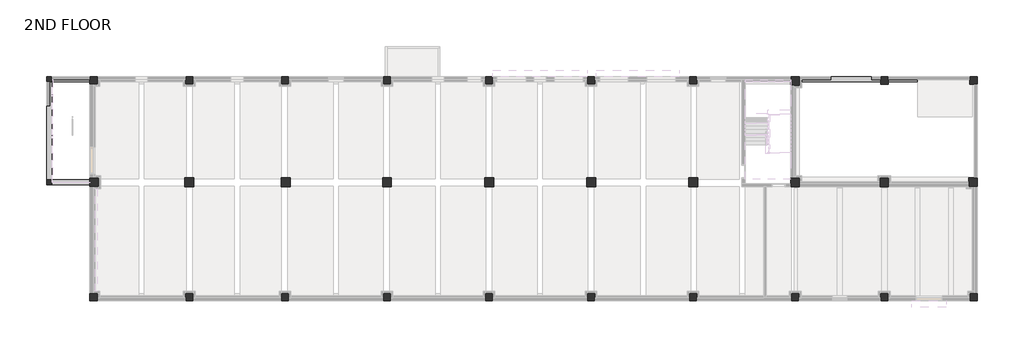
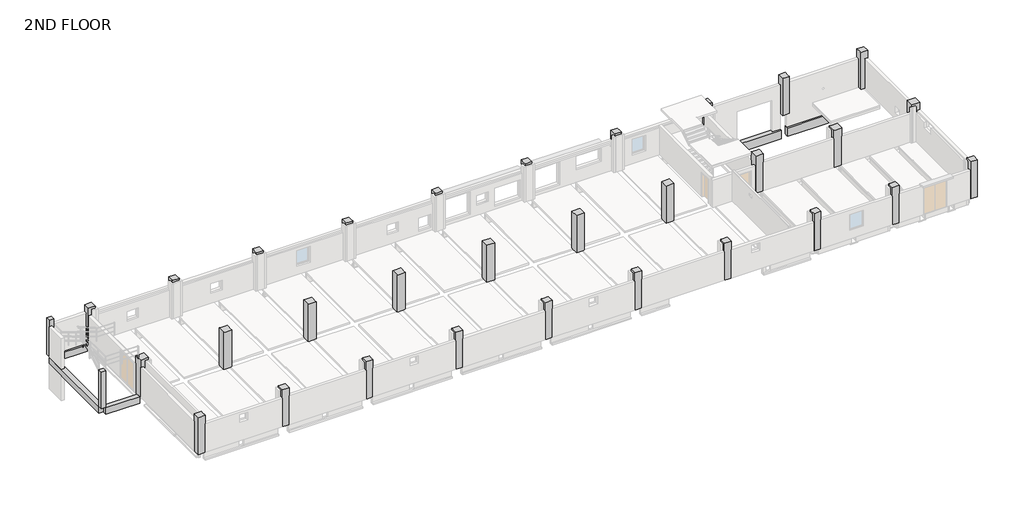
# One storey, part 5 of 7: 32 columns, 8 beams.
"""IFC4 building model written with IfcOpenShell, lengths in millimetres."""

from ifc_helpers import new_model, si_unit, frame, origin, place, context, project, spatial, polyline, outline, extrude, faceted_brep, element, save

model = new_model("IFC4")

# Units and contexts
model_context = context("Model", 3, world=origin())
ifc_project = project(units=[si_unit("LENGTHUNIT", "METRE", prefix="MILLI")], contexts=[model_context])

# Site, building, storey
site = spatial("IfcSite", under=ifc_project)
building = spatial("IfcBuilding", under=site)
storey = spatial("IfcBuildingStorey", under=building, Name="2ND FLOOR", Elevation=10600.0)

# Beams
placement = place(None, origin())
element("IfcBeam", 1, ObjectType="RC Beam_Rectangular : H_SB_AR S16_RC Beam-AG_400x800_2WG1", at=placement, inside=storey, context=model_context, shape_type="Brep", body=[
    faceted_brep([(61700.0, -100.0, 9100.0), (61700.0, 50.0, 9100.0), (61700.0, 300.0, 9100.0), (61000.0, 300.0, 9100.0), (57800.0, 300.0, 9100.0), (55350.0, 300.0, 9100.0), (55350.0, 50.0, 9100.0), (55350.0, -100.0, 9100.0), (61700.0, -100.0, 8300.0), (55350.0, -100.0, 8300.0), (61700.0, 300.0, 8300.0), (61700.0, 50.0, 8300.0), (55350.0, 50.0, 8300.0), (55350.0, 300.0, 8300.0)], [[[0, 1, 2, 3, 4, 5, 6, 7]], [[8, 0, 7, 9]], [[10, 11, 8, 9, 12, 13]], [[2, 10, 13, 5, 4, 3]], [[5, 13, 12, 9, 7, 6]], [[2, 1, 0, 8, 11, 10]]]),
])
element("IfcBeam", 2, ObjectType="RC Beam_Rectangular : H_SB_AR S16_RC Beam-AG_400x800_2WG1", at=placement, inside=storey, context=model_context, shape_type="Brep", body=[
    faceted_brep([(68700.0, -100.0, 9100.0), (68700.0, 50.0, 9100.0), (68700.0, 300.0, 9100.0), (62300.0, 300.0, 9100.0), (62300.0, 50.0, 9100.0), (62300.0, -100.0, 9100.0), (64775.0, -100.0, 9100.0), (64793.0, -100.0, 9100.0), (68700.0, -100.0, 8300.0), (62300.0, -100.0, 8300.0), (64775.0, -100.0, 8300.0), (64793.0, -100.0, 8300.0), (68700.0, 300.0, 8300.0), (68700.0, 50.0, 8300.0), (62300.0, 50.0, 8300.0), (62300.0, 300.0, 8300.0)], [[[0, 1, 2, 3, 4, 5, 6, 7]], [[8, 0, 7, 6, 5, 9, 10, 11]], [[12, 13, 8, 11, 10, 9, 14, 15]], [[2, 12, 15, 3]], [[3, 15, 14, 9, 5, 4]], [[2, 1, 0, 8, 13, 12]]]),
])
element("IfcBeam", 3, ObjectType="RC Beam_Rectangular : H_SB_AR S16_RC Beam-AG_400x600_SWG1", at=placement, inside=storey, context=model_context, shape_type="Brep", body=[
    faceted_brep([(-300.0, -100.0, 10550.0), (-300.0, 50.0, 10550.0), (-300.0, 300.0, 10550.0), (-3300.0, 300.0, 10550.0), (-3300.0, 50.0, 10550.0), (-3300.0, -100.0, 10550.0), (-300.0, -100.0, 9950.0), (-3300.0, -100.0, 9950.0), (-300.0, 300.0, 9950.0), (-300.0, 50.0, 9950.0), (-3300.0, 50.0, 9950.0), (-3300.0, 300.0, 9950.0)], [[[0, 1, 2, 3, 4, 5]], [[6, 0, 5, 7]], [[8, 9, 6, 7, 10, 11]], [[2, 8, 11, 3]], [[2, 1, 0, 6, 9, 8]], [[3, 11, 10, 7, 5, 4]]]),
])
element("IfcBeam", 4, ObjectType="RC Beam_Rectangular : H_SB_AR S16_RC Beam-AG_400x600_SWG2", at=placement, inside=storey, context=model_context, shape_type="Brep", body=[
    faceted_brep([(-3700.0, -7800.0, 10550.0), (-3300.0, -7800.0, 10550.0), (-3300.0, -100.0, 10550.0), (-3450.0, -100.0, 10550.0), (-3700.0, -100.0, 10550.0), (-3700.0, -2000.0, 10550.0), (-3300.0, -7800.0, 9950.0), (-3300.0, -100.0, 9950.0), (-3700.0, -7800.0, 9950.0), (-3700.0, -2000.0, 9950.0), (-3700.0, -100.0, 9950.0), (-3450.0, -100.0, 9950.0)], [[[0, 1, 2, 3, 4, 5]], [[1, 6, 7, 2]], [[6, 8, 9, 10, 11, 7]], [[8, 0, 5, 4, 10, 9]], [[1, 0, 8, 6]], [[4, 3, 2, 7, 11, 10]]]),
])
element("IfcBeam", 5, ObjectType="RC Beam_Rectangular : H_SB_AR S16_RC Beam-AG_400x600_SG1", at=placement, inside=storey, context=model_context, shape_type="SweptSolid", body=[
    extrude(outline(polyline([(-300.0, -7800.0), (-300.0, -8200.0), (-3300.0, -8200.0), (-3300.0, -7800.0), (-300.0, -7800.0)])), frame((0.0, 0.0, 9950.0), z_axis=(0.0, 0.0, 1.0), x_axis=(1.0, 0.0, 0.0)), (0.0, 0.0, 1.0), 600.0),
])
element("IfcBeam", 6, ObjectType="RC Beam_Rectangular : H_SB_AR S16_RC Beam-AG_300x500_2CB1", at=placement, inside=storey, context=model_context, shape_type="Brep", body=[
    faceted_brep([(23150.0, 2350.0, 9300.0), (22850.0, 2350.0, 9300.0), (22850.0, 300.0, 9300.0), (23000.0, 300.0, 9300.0), (23150.0, 300.0, 9300.0), (22850.0, 2350.0, 8800.0), (22850.0, 300.0, 8800.0), (23150.0, 2350.0, 8800.0), (23150.0, 300.0, 8800.0), (23150.0, 2350.0, 9150.0), (23150.0, 300.0, 9150.0)], [[[0, 1, 2, 3, 4]], [[1, 5, 6, 2]], [[5, 7, 8, 6]], [[7, 9, 0, 4, 10, 8]], [[4, 3, 2, 6, 8, 10]], [[0, 9, 7, 5, 1]]]),
])
element("IfcBeam", 7, ObjectType="RC Beam_Rectangular : H_SB_AR S16_RC Beam-AG_300x500_2CB1", at=placement, inside=storey, context=model_context, shape_type="Brep", body=[
    faceted_brep([(27150.0, 2350.0, 9300.0), (26850.0, 2350.0, 9300.0), (26850.0, 300.0, 9300.0), (27000.0, 300.0, 9300.0), (27150.0, 300.0, 9300.0), (26850.0, 2350.0, 9150.0), (26850.0, 2350.0, 8800.0), (26850.0, 300.0, 8800.0), (26850.0, 300.0, 9150.0), (27150.0, 2350.0, 8800.0), (27150.0, 300.0, 8800.0)], [[[0, 1, 2, 3, 4]], [[1, 5, 6, 7, 8, 2]], [[6, 9, 10, 7]], [[9, 0, 4, 10]], [[4, 3, 2, 8, 7, 10]], [[0, 9, 6, 5, 1]]]),
])
element("IfcBeam", 8, ObjectType="RC Beam_Rectangular : H_SB_AR S16_RC Beam-AG_300x500_2CB2", at=placement, inside=storey, context=model_context, shape_type="Brep", body=[
    faceted_brep([(26850.0, 2350.0, 9300.0), (26850.0, 2650.0, 9300.0), (23150.0, 2650.0, 9300.0), (23150.0, 2350.0, 9300.0), (26850.0, 2350.0, 8800.0), (26850.0, 2350.0, 9150.0), (23150.0, 2350.0, 9150.0), (23150.0, 2350.0, 8800.0), (26850.0, 2650.0, 8800.0), (23150.0, 2650.0, 8800.0)], [[[0, 1, 2, 3]], [[4, 5, 0, 3, 6, 7]], [[8, 4, 7, 9]], [[1, 8, 9, 2]], [[2, 9, 7, 6, 3]], [[1, 0, 5, 4, 8]]]),
])

# Columns
element("IfcColumn", 9, ObjectType="RC_Column_Rectangular : H_SC_AR S15_RC Col-AG_700x700_C1", at=placement, inside=storey, context=model_context, shape_type="Brep", body=[
    faceted_brep([(400.0, -7650.0, 10600.0), (400.0, -7700.0, 10600.0), (400.0, -8300.0, 10600.0), (400.0, -8350.0, 10600.0), (399.4974747, -8350.0, 10600.0), (-50.0, -8350.0, 10600.0), (-300.0, -8350.0, 10600.0), (-300.0, -7650.0, 10600.0), (-50.0, -7650.0, 10600.0), (399.4974747, -7650.0, 10600.0), (400.0, -7650.0, 13920.0), (400.0, -7700.0, 13920.0), (400.0, -7700.0, 14100.0), (400.0, -8300.0, 14100.0), (400.0, -8300.0, 13920.0), (400.0, -8350.0, 13920.0), (399.4974747, -8350.0, 13920.0), (399.4974747, -8350.0, 14100.0), (100.0, -8350.0, 14100.0), (-300.0, -8350.0, 14100.0), (-300.0, -8350.0, 13400.0), (-300.0, -7650.0, 14100.0), (-300.0, -7650.0, 13400.0), (100.0, -7650.0, 14100.0), (399.4974747, -7650.0, 14100.0), (399.4974747, -7650.0, 13920.0), (399.4974747, -8300.0, 14100.0), (399.4974747, -7700.0, 14100.0), (399.4974747, -7700.0, 13920.0), (399.4974747, -8300.0, 13920.0)], [[[0, 1, 2, 3, 4, 5, 6, 7, 8, 9]], [[3, 2, 1, 0, 10, 11, 12, 13, 14, 15]], [[6, 5, 4, 3, 15, 16, 17, 18, 19, 20]], [[7, 6, 20, 19, 21, 22]], [[0, 9, 8, 7, 22, 21, 23, 24, 25, 10]], [[21, 19, 18, 17, 26, 13, 12, 27, 24, 23]], [[25, 28, 11, 10]], [[28, 27, 12, 11]], [[28, 25, 24, 27]], [[16, 29, 26, 17]], [[26, 29, 14, 13]], [[29, 16, 15, 14]]]),
])
element("IfcColumn", 10, ObjectType="RC_Column_Rectangular : H_SC_AR S15_RC Col-AG_700x700_C1", at=placement, inside=storey, context=model_context, shape_type="Brep", body=[
    faceted_brep([(7850.0, -7650.0, 10600.0), (7850.0, -8350.0, 10600.0), (7150.0, -8350.0, 10600.0), (7150.0, -7650.0, 10600.0), (7850.0, -7650.0, 13920.0), (7850.0, -7650.0, 14100.0), (7850.0, -7700.0, 14100.0), (7850.0, -8300.0, 14100.0), (7850.0, -8350.0, 14100.0), (7850.0, -8350.0, 13920.0), (7750.0, -8350.0, 14100.0), (7250.0, -8350.0, 14100.0), (7150.0, -8350.0, 14100.0), (7150.0, -8350.0, 13920.0), (7150.0, -8300.0, 14100.0), (7150.0, -7700.0, 14100.0), (7150.0, -7650.0, 14100.0), (7150.0, -7650.0, 13920.0), (7250.0, -7650.0, 14100.0), (7750.0, -7650.0, 14100.0)], [[[0, 1, 2, 3]], [[1, 0, 4, 5, 6, 7, 8, 9]], [[2, 1, 9, 8, 10, 11, 12, 13]], [[3, 2, 13, 12, 14, 15, 16, 17]], [[0, 3, 17, 16, 18, 19, 5, 4]], [[18, 16, 15, 14, 12, 11, 10, 8, 7, 6, 5, 19]]]),
])
element("IfcColumn", 11, ObjectType="RC_Column_Rectangular : H_SC_AR S15_RC Col-AG_700x700_C1", at=placement, inside=storey, context=model_context, shape_type="Brep", body=[
    faceted_brep([(15400.0000001, -7650.0, 10600.0), (15400.0000001, -8350.0, 10600.0), (14700.0000001, -8350.0, 10600.0), (14700.0000001, -7650.0, 10600.0), (15400.0000001, -7650.0, 13920.0), (15400.0000001, -7650.0, 14100.0), (15400.0000001, -7700.0, 14100.0), (15400.0000001, -8300.0, 14100.0), (15400.0000001, -8350.0, 14100.0), (15400.0000001, -8350.0, 13920.0), (15250.0, -8350.0, 14100.0), (14750.0, -8350.0, 14100.0), (14700.0000001, -8350.0, 14100.0), (14700.0000001, -8350.0, 13920.0), (14700.0000001, -8300.0, 14100.0), (14700.0000001, -7700.0, 14100.0), (14700.0000001, -7650.0, 14100.0), (14700.0000001, -7650.0, 13920.0), (14750.0, -7650.0, 14100.0), (15250.0, -7650.0, 14100.0)], [[[0, 1, 2, 3]], [[1, 0, 4, 5, 6, 7, 8, 9]], [[2, 1, 9, 8, 10, 11, 12, 13]], [[3, 2, 13, 12, 14, 15, 16, 17]], [[0, 3, 17, 16, 18, 19, 5, 4]], [[5, 19, 18, 16, 15, 14, 12, 11, 10, 8, 7, 6]]]),
])
element("IfcColumn", 12, ObjectType="RC_Column_Rectangular : H_SC_AR S15_RC Col-AG_700x700_C1", at=placement, inside=storey, context=model_context, shape_type="Brep", body=[
    faceted_brep([(23350.0000003, -7650.0, 10600.0), (23350.0000003, -8350.0, 10600.0), (22650.0000003, -8350.0, 10600.0), (22650.0000003, -7650.0, 10600.0), (23350.0000003, -7650.0, 13920.0), (23350.0000003, -7650.0, 14100.0), (23350.0000003, -7700.0, 14100.0), (23350.0000003, -8300.0, 14100.0), (23350.0000003, -8350.0, 14100.0), (23350.0000003, -8350.0, 13920.0), (23250.0, -8350.0, 14100.0), (22750.0, -8350.0, 14100.0), (22650.0000003, -8350.0, 14100.0), (22650.0000003, -8350.0, 13920.0), (22650.0000003, -8300.0, 14100.0), (22650.0000003, -7700.0, 14100.0), (22650.0000003, -7650.0, 14100.0), (22650.0000003, -7650.0, 13920.0), (22750.0, -7650.0, 14100.0), (23250.0, -7650.0, 14100.0)], [[[0, 1, 2, 3]], [[1, 0, 4, 5, 6, 7, 8, 9]], [[2, 1, 9, 8, 10, 11, 12, 13]], [[3, 2, 13, 12, 14, 15, 16, 17]], [[0, 3, 17, 16, 18, 19, 5, 4]], [[18, 16, 15, 14, 12, 11, 10, 8, 7, 6, 5, 19]]]),
])
element("IfcColumn", 13, ObjectType="RC_Column_Rectangular : H_SC_AR S15_RC Col-AG_700x700_C1", at=placement, inside=storey, context=model_context, shape_type="Brep", body=[
    faceted_brep([(31350.0000002, -7650.0, 10600.0), (31350.0000002, -8350.0, 10600.0), (30650.0000002, -8350.0, 10600.0), (30650.0000002, -7650.0, 10600.0), (31350.0000002, -7650.0, 13920.0), (31350.0000002, -7650.0, 14100.0), (31350.0000002, -7700.0, 14100.0), (31350.0000002, -8300.0, 14100.0), (31350.0000002, -8350.0, 14100.0), (31350.0000002, -8350.0, 13920.0), (31249.9999998, -8350.0, 14100.0), (30750.0000002, -8350.0, 14100.0), (30650.0000002, -8350.0, 14100.0), (30650.0000002, -8350.0, 13920.0), (30650.0000002, -8300.0, 14100.0), (30650.0000002, -7700.0, 14100.0), (30650.0000002, -7650.0, 14100.0), (30650.0000002, -7650.0, 13920.0), (30750.0000002, -7650.0, 14100.0), (31249.9999998, -7650.0, 14100.0)], [[[0, 1, 2, 3]], [[1, 0, 4, 5, 6, 7, 8, 9]], [[2, 1, 9, 8, 10, 11, 12, 13]], [[3, 2, 13, 12, 14, 15, 16, 17]], [[0, 3, 17, 16, 18, 19, 5, 4]], [[18, 16, 15, 14, 12, 11, 10, 8, 7, 6, 5, 19]]]),
])
element("IfcColumn", 14, ObjectType="RC_Column_Rectangular : H_SC_AR S15_RC Col-AG_700x700_C1", at=placement, inside=storey, context=model_context, shape_type="Brep", body=[
    faceted_brep([(39350.0000001, -7650.0, 10600.0), (39350.0000001, -8350.0, 10600.0), (38650.0000001, -8350.0, 10600.0), (38650.0000001, -7650.0, 10600.0), (39350.0000001, -7650.0, 13920.0), (39350.0000001, -7650.0, 14100.0), (39350.0000001, -7700.0, 14100.0), (39350.0000001, -8300.0, 14100.0), (39350.0000001, -8350.0, 14100.0), (39350.0000001, -8350.0, 13920.0), (39249.9999998, -8350.0, 14100.0), (38750.0000002, -8350.0, 14100.0), (38650.0000001, -8350.0, 14100.0), (38650.0000001, -8350.0, 13920.0), (38650.0000001, -8300.0, 14100.0), (38650.0000001, -7700.0, 14100.0), (38650.0000001, -7650.0, 14100.0), (38650.0000001, -7650.0, 13920.0), (38750.0000002, -7650.0, 14100.0), (39249.9999998, -7650.0, 14100.0)], [[[0, 1, 2, 3]], [[1, 0, 4, 5, 6, 7, 8, 9]], [[2, 1, 9, 8, 10, 11, 12, 13]], [[3, 2, 13, 12, 14, 15, 16, 17]], [[0, 3, 17, 16, 18, 19, 5, 4]], [[18, 16, 15, 14, 12, 11, 10, 8, 7, 6, 5, 19]]]),
])
element("IfcColumn", 15, ObjectType="RC_Column_Rectangular : H_SC_AR S15_RC Col-AG_700x700_C1", at=placement, inside=storey, context=model_context, shape_type="Brep", body=[
    faceted_brep([(47349.9999999, -7650.0, 10600.0), (47349.9999999, -8350.0, 10600.0), (46649.9999999, -8350.0, 10600.0), (46649.9999999, -7650.0, 10600.0), (47349.9999999, -7650.0, 13920.0), (47349.9999999, -7650.0, 14100.0), (47349.9999999, -7750.0, 14100.0), (47349.9999999, -8350.0, 14100.0), (47349.9999999, -8350.0, 13920.0), (47250.0, -8350.0, 14100.0), (46750.0, -8350.0, 14100.0), (46649.9999999, -8350.0, 14100.0), (46649.9999999, -8350.0, 13920.0), (46649.9999999, -8300.0, 14100.0), (46649.9999999, -7700.0, 14100.0), (46649.9999999, -7650.0, 14100.0), (46649.9999999, -7650.0, 13920.0), (46750.0, -7650.0, 14100.0), (47250.0, -7650.0, 14100.0)], [[[0, 1, 2, 3]], [[1, 0, 4, 5, 6, 7, 8]], [[2, 1, 8, 7, 9, 10, 11, 12]], [[3, 2, 12, 11, 13, 14, 15, 16]], [[0, 3, 16, 15, 17, 18, 5, 4]], [[17, 15, 14, 13, 11, 10, 9, 7, 6, 5, 18]]]),
])
element("IfcColumn", 16, ObjectType="RC_Column_Rectangular : H_SC_AR S15_RC Col-AG_700x700_C1", at=placement, inside=storey, context=model_context, shape_type="Brep", body=[
    faceted_brep([(55350.0, -7650.0, 10600.0), (55350.0, -8100.0, 10600.0), (55350.0, -8350.0, 10600.0), (54650.0, -8350.0, 10600.0), (54650.0, -8100.0, 10600.0), (54650.0, -7650.0, 10600.0), (54900.0, -7650.0, 10600.0), (55350.0, -7650.0, 13920.0), (55350.0, -7650.0, 14100.0), (55350.0, -7750.0, 14100.0), (55350.0, -8350.0, 14100.0), (55350.0, -8350.0, 13920.0), (55350.0, -8350.0, 13300.0), (55200.0, -8350.0, 14100.0), (54700.0, -8350.0, 14100.0), (54650.0, -8350.0, 14100.0), (54650.0, -8350.0, 13920.0), (54650.0, -8350.0, 13200.0), (54650.0, -7650.0, 14100.0), (54650.0, -7650.0, 13300.0), (55150.0, -7650.0, 14100.0)], [[[0, 1, 2, 3, 4, 5, 6]], [[2, 1, 0, 7, 8, 9, 10, 11, 12]], [[3, 2, 12, 11, 10, 13, 14, 15, 16, 17]], [[5, 4, 3, 17, 16, 15, 18, 19]], [[0, 6, 5, 19, 18, 20, 8, 7]], [[18, 15, 14, 13, 10, 9, 8, 20]]]),
])
element("IfcColumn", 17, ObjectType="RC_Column_Rectangular : H_SC_AR S15_RC Col-AG_700x700_C1", at=placement, inside=storey, context=model_context, shape_type="Brep", body=[
    faceted_brep([(62350.0, -7650.0, 10600.0), (62350.0, -8100.0, 10600.0), (62350.0, -8350.0, 10600.0), (61650.0, -8350.0, 10600.0), (61650.0, -8100.0, 10600.0), (61650.0, -7650.0, 10600.0), (62350.0, -7650.0, 13920.0), (62350.0, -7650.0, 14100.0), (62350.0, -7750.0, 14100.0), (62350.0, -8350.0, 14100.0), (62350.0, -8350.0, 13920.0), (62350.0, -8350.0, 13300.0), (62250.0, -8350.0, 14100.0), (61750.0, -8350.0, 14100.0), (61650.0, -8350.0, 14100.0), (61650.0, -8350.0, 13920.0), (61650.0, -8350.0, 13300.0), (61650.0, -7750.0, 14100.0), (61650.0, -7650.0, 14100.0), (61650.0, -7650.0, 13920.0), (61750.0, -7650.0, 14100.0), (62250.0, -7650.0, 14100.0)], [[[0, 1, 2, 3, 4, 5]], [[2, 1, 0, 6, 7, 8, 9, 10, 11]], [[3, 2, 11, 10, 9, 12, 13, 14, 15, 16]], [[5, 4, 3, 16, 15, 14, 17, 18, 19]], [[0, 5, 19, 18, 20, 21, 7, 6]], [[20, 18, 17, 14, 13, 12, 9, 8, 7, 21]]]),
])
element("IfcColumn", 18, ObjectType="RC_Column_Rectangular : H_SC_AR S15_RC Col-AG_700x700_C1", at=placement, inside=storey, context=model_context, shape_type="Brep", body=[
    faceted_brep([(69300.0, -7650.0, 10600.0), (69300.0, -8350.0, 10600.0), (69050.0, -8350.0, 10600.0), (68600.0, -8350.0, 10600.0), (68600.0, -8100.0, 10600.0), (68600.0, -7650.0, 10600.0), (69050.0, -7650.0, 10600.0), (69300.0, -7650.0, 13400.0), (69300.0, -7650.0, 14100.0), (69300.0, -8350.0, 14100.0), (69300.0, -8350.0, 13400.0), (68900.0, -8350.0, 14100.0), (68600.0, -8350.0, 14100.0), (68600.0, -8350.0, 13920.0), (68600.0, -8350.0, 13300.0), (68600.0, -7750.0, 14100.0), (68600.0, -7650.0, 14100.0), (68600.0, -7650.0, 13920.0), (68900.0, -7650.0, 14100.0)], [[[0, 1, 2, 3, 4, 5, 6]], [[1, 0, 7, 8, 9, 10]], [[3, 2, 1, 10, 9, 11, 12, 13, 14]], [[5, 4, 3, 14, 13, 12, 15, 16, 17]], [[0, 6, 5, 17, 16, 18, 8, 7]], [[9, 8, 18, 16, 15, 12, 11]]]),
])
element("IfcColumn", 19, ObjectType="RC_Column_Rectangular : H_SC_AR S15_RC Col-AG_700x700_C1", at=placement, inside=storey, context=model_context, shape_type="Brep", body=[
    faceted_brep([(55350.0, 300.0, 10600.0), (55350.0, -400.0, 10600.0), (54900.0, -400.0, 10600.0), (54650.0, -400.0, 10600.0), (54650.0, 50.0, 10600.0), (54650.0, 300.0, 10600.0), (55350.0, 300.0, 13300.0), (55350.0, 300.0, 14100.0), (55350.0, -100.0, 14100.0), (55350.0, -400.0, 14100.0), (55350.0, -400.0, 13920.0), (55150.0, -400.0, 14100.0), (54900.0, -400.0, 14100.0), (54650.0, -400.0, 14100.0), (54650.0, -400.0, 13300.0), (54650.0, -387.0, 14100.0), (54650.0, 300.0, 14100.0), (54650.0, 300.0, 13300.0)], [[[0, 1, 2, 3, 4, 5]], [[1, 0, 6, 7, 8, 9, 10]], [[3, 2, 1, 10, 9, 11, 12, 13, 14]], [[5, 4, 3, 14, 13, 15, 16, 17]], [[0, 5, 17, 16, 7, 6]], [[16, 15, 13, 12, 11, 9, 8, 7]]]),
])
element("IfcColumn", 20, ObjectType="RC_Column_Rectangular : H_SC_AR S15_RC Col-AG_600x600_C2", at=placement, inside=storey, context=model_context, shape_type="Brep", body=[
    faceted_brep([(300.0, 300.0, 10600.0), (300.0, 50.0, 10600.0), (300.0, -300.0, 10600.0), (-50.0, -300.0, 10600.0), (-300.0, -300.0, 10600.0), (-300.0, 300.0, 10600.0), (300.0, 300.0, 13300.0), (300.0, 300.0, 14100.0), (300.0, -100.0, 14100.0), (300.0, -300.0, 14100.0), (300.0, -300.0, 13920.0), (100.0, -300.0, 14100.0), (-300.0, -300.0, 14100.0), (-300.0, -300.0, 13400.0), (-300.0, 300.0, 14100.0), (-300.0, 300.0, 14050.0), (-300.0, 300.0, 13450.0)], [[[0, 1, 2, 3, 4, 5]], [[2, 1, 0, 6, 7, 8, 9, 10]], [[4, 3, 2, 10, 9, 11, 12, 13]], [[5, 4, 13, 12, 14, 15, 16]], [[0, 5, 16, 15, 14, 7, 6]], [[14, 12, 11, 9, 8, 7]]]),
])
element("IfcColumn", 21, ObjectType="RC_Column_Rectangular : H_SC_AR S15_RC Col-AG_600x600_C2", at=placement, inside=storey, context=model_context, shape_type="Brep", body=[
    faceted_brep([(7800.0, 300.0, 10600.0), (7800.0, 50.0, 10600.0), (7800.0, -300.0, 10600.0), (7200.0, -300.0, 10600.0), (7200.0, 50.0, 10600.0), (7200.0, 300.0, 10600.0), (7800.0, 300.0, 13300.0), (7800.0, 300.0, 14100.0), (7800.0, -100.0, 14100.0), (7800.0, -300.0, 14100.0), (7800.0, -300.0, 13920.0), (7750.0, -300.0, 14100.0), (7250.0, -300.0, 14100.0), (7200.0, -300.0, 14100.0), (7200.0, -300.0, 13920.0), (7200.0, -100.0, 14100.0), (7200.0, 300.0, 14100.0), (7200.0, 300.0, 13300.0)], [[[0, 1, 2, 3, 4, 5]], [[2, 1, 0, 6, 7, 8, 9, 10]], [[3, 2, 10, 9, 11, 12, 13, 14]], [[5, 4, 3, 14, 13, 15, 16, 17]], [[0, 5, 17, 16, 7, 6]], [[7, 16, 15, 13, 12, 11, 9, 8]]]),
])
element("IfcColumn", 22, ObjectType="RC_Column_Rectangular : H_SC_AR S15_RC Col-AG_600x600_C2", at=placement, inside=storey, context=model_context, shape_type="Brep", body=[
    faceted_brep([(15300.0, 300.0, 10600.0), (15300.0, 50.0, 10600.0), (15300.0, -300.0, 10600.0), (14700.0, -300.0, 10600.0), (14700.0, 50.0, 10600.0), (14700.0, 300.0, 10600.0), (15300.0, 300.0, 13300.0), (15300.0, 300.0, 14100.0), (15300.0, -100.0, 14100.0), (15300.0, -300.0, 14100.0), (15300.0, -300.0, 13920.0), (15250.0, -300.0, 14100.0), (14750.0, -300.0, 14100.0), (14700.0, -300.0, 14100.0), (14700.0, -300.0, 13920.0), (14700.0, -100.0, 14100.0), (14700.0, 300.0, 14100.0), (14700.0, 300.0, 13300.0)], [[[0, 1, 2, 3, 4, 5]], [[2, 1, 0, 6, 7, 8, 9, 10]], [[3, 2, 10, 9, 11, 12, 13, 14]], [[5, 4, 3, 14, 13, 15, 16, 17]], [[0, 5, 17, 16, 7, 6]], [[7, 16, 15, 13, 12, 11, 9, 8]]]),
])
element("IfcColumn", 23, ObjectType="RC_Column_Rectangular : H_SC_AR S15_RC Col-AG_600x600_C2", at=placement, inside=storey, context=model_context, shape_type="Brep", body=[
    faceted_brep([(23300.0, 300.0, 10600.0), (23300.0, 50.0, 10600.0), (23300.0, -300.0, 10600.0), (22700.0, -300.0, 10600.0), (22700.0, 50.0, 10600.0), (22700.0, 300.0, 10600.0), (23300.0, 300.0, 13300.0), (23300.0, 300.0, 14100.0), (23300.0, -100.0, 14100.0), (23300.0, -300.0, 14100.0), (23300.0, -300.0, 13920.0), (23250.0, -300.0, 14100.0), (22750.0, -300.0, 14100.0), (22700.0, -300.0, 14100.0), (22700.0, -300.0, 13920.0), (22700.0, -100.0, 14100.0), (22700.0, 300.0, 14100.0), (22700.0, 300.0, 13300.0)], [[[0, 1, 2, 3, 4, 5]], [[2, 1, 0, 6, 7, 8, 9, 10]], [[3, 2, 10, 9, 11, 12, 13, 14]], [[5, 4, 3, 14, 13, 15, 16, 17]], [[0, 5, 17, 16, 7, 6]], [[7, 16, 15, 13, 12, 11, 9, 8]]]),
])
element("IfcColumn", 24, ObjectType="RC_Column_Rectangular : H_SC_AR S15_RC Col-AG_600x600_C2", at=placement, inside=storey, context=model_context, shape_type="Brep", body=[
    faceted_brep([(31300.0, 300.0, 10600.0), (31300.0, 50.0, 10600.0), (31300.0, -300.0, 10600.0), (30700.0, -300.0, 10600.0), (30700.0, 50.0, 10600.0), (30700.0, 300.0, 10600.0), (31300.0, 300.0, 13300.0), (31300.0, 300.0, 14100.0), (31300.0, -100.0, 14100.0), (31300.0, -300.0, 14100.0), (31300.0, -300.0, 13920.0), (31249.9999998, -300.0, 14100.0), (30750.0000002, -300.0, 14100.0), (30700.0, -300.0, 14100.0), (30700.0, -300.0, 13920.0), (30700.0, -100.0, 14100.0), (30700.0, 300.0, 14100.0), (30700.0, 300.0, 13300.0)], [[[0, 1, 2, 3, 4, 5]], [[2, 1, 0, 6, 7, 8, 9, 10]], [[3, 2, 10, 9, 11, 12, 13, 14]], [[5, 4, 3, 14, 13, 15, 16, 17]], [[0, 5, 17, 16, 7, 6]], [[7, 16, 15, 13, 12, 11, 9, 8]]]),
])
element("IfcColumn", 25, ObjectType="RC_Column_Rectangular : H_SC_AR S15_RC Col-AG_600x600_C2", at=placement, inside=storey, context=model_context, shape_type="Brep", body=[
    faceted_brep([(39300.0, 300.0, 10600.0), (39300.0, 50.0, 10600.0), (39300.0, -300.0, 10600.0), (38700.0, -300.0, 10600.0), (38700.0, 50.0, 10600.0), (38700.0, 300.0, 10600.0), (39300.0, 300.0, 13300.0), (39300.0, 300.0, 14100.0), (39300.0, -100.0, 14100.0), (39300.0, -300.0, 14100.0), (39300.0, -300.0, 13920.0), (39249.9999998, -300.0, 14100.0), (38750.0000002, -300.0, 14100.0), (38700.0, -300.0, 14100.0), (38700.0, -300.0, 13920.0), (38700.0, -100.0, 14100.0), (38700.0, 300.0, 14100.0), (38700.0, 300.0, 13300.0)], [[[0, 1, 2, 3, 4, 5]], [[2, 1, 0, 6, 7, 8, 9, 10]], [[3, 2, 10, 9, 11, 12, 13, 14]], [[5, 4, 3, 14, 13, 15, 16, 17]], [[0, 5, 17, 16, 7, 6]], [[7, 16, 15, 13, 12, 11, 9, 8]]]),
])
element("IfcColumn", 26, ObjectType="RC_Column_Rectangular : H_SC_AR S15_RC Col-AG_600x600_C2", at=placement, inside=storey, context=model_context, shape_type="Brep", body=[
    faceted_brep([(47300.0, 300.0, 10600.0), (47300.0, 50.0, 10600.0), (47300.0, -300.0, 10600.0), (46700.0, -300.0, 10600.0), (46700.0, 50.0, 10600.0), (46700.0, 300.0, 10600.0), (47300.0, 300.0, 13300.0), (47300.0, 300.0, 14100.0), (47300.0, -100.0, 14100.0), (47300.0, -300.0, 14100.0), (47300.0, -300.0, 13920.0), (47250.0, -300.0, 14100.0), (46750.0, -300.0, 14100.0), (46700.0, -300.0, 14100.0), (46700.0, -300.0, 13920.0), (46700.0, -100.0, 14100.0), (46700.0, 300.0, 14100.0), (46700.0, 300.0, 13300.0)], [[[0, 1, 2, 3, 4, 5]], [[2, 1, 0, 6, 7, 8, 9, 10]], [[3, 2, 10, 9, 11, 12, 13, 14]], [[5, 4, 3, 14, 13, 15, 16, 17]], [[0, 5, 17, 16, 7, 6]], [[7, 16, 15, 13, 12, 11, 9, 8]]]),
])
element("IfcColumn", 27, ObjectType="RC_Column_Rectangular : H_SC_AR S15_RC Col-AG_600x600_C2", at=placement, inside=storey, context=model_context, shape_type="Brep", body=[
    faceted_brep([(62300.0, 300.0, 10600.0), (62300.0, -300.0, 10600.0), (61700.0, -300.0, 10600.0), (61700.0, 300.0, 10600.0), (62300.0, 300.0, 13300.0), (62300.0, 300.0, 14100.0), (62300.0, -100.0, 14100.0), (62300.0, -300.0, 14100.0), (62300.0, -300.0, 13920.0), (62250.0, -300.0, 14100.0), (61750.0, -300.0, 14100.0), (61700.0, -300.0, 14100.0), (61700.0, -300.0, 13920.0), (61700.0, -100.0, 14100.0), (61700.0, 300.0, 14100.0), (61700.0, 300.0, 13300.0)], [[[0, 1, 2, 3]], [[1, 0, 4, 5, 6, 7, 8]], [[2, 1, 8, 7, 9, 10, 11, 12]], [[3, 2, 12, 11, 13, 14, 15]], [[0, 3, 15, 14, 5, 4]], [[5, 14, 13, 11, 10, 9, 7, 6]]]),
])
element("IfcColumn", 28, ObjectType="RC_Column_Rectangular : H_SC_AR S15_RC Col-AG_600x600_C2", at=placement, inside=storey, context=model_context, shape_type="Brep", body=[
    faceted_brep([(69300.0, 300.0, 10600.0), (69300.0, -300.0, 10600.0), (69050.0, -300.0, 10600.0), (68700.0, -300.0, 10600.0), (68700.0, 300.0, 10600.0), (69300.0, 300.0, 14100.0), (69300.0, -300.0, 14100.0), (69300.0, -300.0, 13400.0), (68900.0, -300.0, 14100.0), (68700.0, -300.0, 14100.0), (68700.0, -300.0, 13920.0), (68700.0, -100.0, 14100.0), (68700.0, 300.0, 14100.0), (68700.0, 300.0, 13300.0)], [[[0, 1, 2, 3, 4]], [[1, 0, 5, 6, 7]], [[3, 2, 1, 7, 6, 8, 9, 10]], [[4, 3, 10, 9, 11, 12, 13]], [[0, 4, 13, 12, 5]], [[6, 5, 12, 11, 9, 8]]]),
])
element("IfcColumn", 29, ObjectType="RC_Column_Rectangular : H_SC_AR S15_RC Col-AG_600x600_C2", at=placement, inside=storey, context=model_context, shape_type="Brep", body=[
    faceted_brep([(69300.0, -16700.0, 10600.0), (69300.0, -17300.0, 10600.0), (68700.0, -17300.0, 10600.0), (68700.0, -17050.0, 10600.0), (68700.0, -16700.0, 10600.0), (69050.0, -16700.0, 10600.0), (69300.0, -16700.0, 13400.0), (69300.0, -16700.0, 14100.0), (69300.0, -17300.0, 14100.0), (68700.0, -17300.0, 14100.0), (68700.0, -17300.0, 13300.0), (68700.0, -16900.0, 14100.0), (68700.0, -16700.0, 14100.0), (68700.0, -16700.0, 13920.0), (68900.0, -16700.0, 14100.0)], [[[0, 1, 2, 3, 4, 5]], [[1, 0, 6, 7, 8]], [[2, 1, 8, 9, 10]], [[4, 3, 2, 10, 9, 11, 12, 13]], [[0, 5, 4, 13, 12, 14, 7, 6]], [[8, 7, 14, 12, 11, 9]]]),
])
element("IfcColumn", 30, ObjectType="RC_Column_Rectangular : H_SC_AR S15_RC Col-AG_600x600_C2", at=placement, inside=storey, context=model_context, shape_type="Brep", body=[
    faceted_brep([(62300.0, -16700.0, 10600.0), (62300.0, -17050.0, 10600.0), (62300.0, -17300.0, 10600.0), (61700.0, -17300.0, 10600.0), (61700.0, -17050.0, 10600.0), (61700.0, -16700.0, 10600.0), (62300.0, -16700.0, 13920.0), (62300.0, -16700.0, 14100.0), (62300.0, -16900.0, 14100.0), (62300.0, -17300.0, 14100.0), (62300.0, -17300.0, 13300.0), (61700.0, -17300.0, 14100.0), (61700.0, -17300.0, 13300.0), (61700.0, -16900.0, 14100.0), (61700.0, -16700.0, 14100.0), (61700.0, -16700.0, 13920.0), (61750.0, -16700.0, 14100.0), (62250.0, -16700.0, 14100.0)], [[[0, 1, 2, 3, 4, 5]], [[2, 1, 0, 6, 7, 8, 9, 10]], [[3, 2, 10, 9, 11, 12]], [[5, 4, 3, 12, 11, 13, 14, 15]], [[0, 5, 15, 14, 16, 17, 7, 6]], [[11, 9, 8, 7, 17, 16, 14, 13]]]),
])
element("IfcColumn", 31, ObjectType="RC_Column_Rectangular : H_SC_AR S15_RC Col-AG_600x600_C2", at=placement, inside=storey, context=model_context, shape_type="Brep", body=[
    faceted_brep([(55300.0, -16700.0, 10600.0), (55300.0, -17050.0, 10600.0), (55300.0, -17300.0, 10600.0), (54700.0, -17300.0, 10600.0), (54700.0, -17050.0, 10600.0), (54700.0, -16700.0, 10600.0), (55300.0, -16700.0, 13920.0), (55300.0, -16700.0, 14100.0), (55300.0, -16900.0, 14100.0), (55300.0, -17300.0, 14100.0), (55300.0, -17300.0, 13300.0), (54700.0, -17300.0, 14100.0), (54700.0, -17300.0, 13300.0), (54700.0, -16900.0, 14100.0), (54700.0, -16700.0, 14100.0), (54700.0, -16700.0, 13920.0), (55200.0, -16700.0, 14100.0)], [[[0, 1, 2, 3, 4, 5]], [[2, 1, 0, 6, 7, 8, 9, 10]], [[3, 2, 10, 9, 11, 12]], [[5, 4, 3, 12, 11, 13, 14, 15]], [[0, 5, 15, 14, 16, 7, 6]], [[11, 9, 8, 7, 16, 14, 13]]]),
])
element("IfcColumn", 32, ObjectType="RC_Column_Rectangular : H_SC_AR S15_RC Col-AG_600x600_C2", at=placement, inside=storey, context=model_context, shape_type="Brep", body=[
    faceted_brep([(46700.0, -16700.0, 10600.0), (47300.0, -16700.0, 10600.0), (47300.0, -17050.0, 10600.0), (47300.0, -17300.0, 10600.0), (46700.0, -17300.0, 10600.0), (46700.0, -17050.0, 10600.0), (46700.0, -16700.0, 13920.0), (46700.0, -16700.0, 14100.0), (46750.0, -16700.0, 14100.0), (47250.0, -16700.0, 14100.0), (47300.0, -16700.0, 14100.0), (47300.0, -16700.0, 13920.0), (47300.0, -16900.0, 14100.0), (47300.0, -17300.0, 14100.0), (47300.0, -17300.0, 13300.0), (46700.0, -17300.0, 14100.0), (46700.0, -17300.0, 13300.0), (46700.0, -16900.0, 14100.0)], [[[0, 1, 2, 3, 4, 5]], [[1, 0, 6, 7, 8, 9, 10, 11]], [[3, 2, 1, 11, 10, 12, 13, 14]], [[4, 3, 14, 13, 15, 16]], [[0, 5, 4, 16, 15, 17, 7, 6]], [[15, 13, 12, 10, 9, 8, 7, 17]]]),
])
element("IfcColumn", 33, ObjectType="RC_Column_Rectangular : H_SC_AR S15_RC Col-AG_600x600_C2", at=placement, inside=storey, context=model_context, shape_type="Brep", body=[
    faceted_brep([(38700.0, -16700.0, 10600.0), (39300.0, -16700.0, 10600.0), (39300.0, -17050.0, 10600.0), (39300.0, -17300.0, 10600.0), (38700.0, -17300.0, 10600.0), (38700.0, -17050.0, 10600.0), (38700.0, -16700.0, 13920.0), (38700.0, -16700.0, 14100.0), (38750.0000002, -16700.0, 14100.0), (39249.9999998, -16700.0, 14100.0), (39300.0, -16700.0, 14100.0), (39300.0, -16700.0, 13920.0), (39300.0, -16900.0, 14100.0), (39300.0, -17300.0, 14100.0), (39300.0, -17300.0, 13300.0), (38700.0, -17300.0, 14100.0), (38700.0, -17300.0, 13300.0), (38700.0, -16900.0, 14100.0)], [[[0, 1, 2, 3, 4, 5]], [[1, 0, 6, 7, 8, 9, 10, 11]], [[3, 2, 1, 11, 10, 12, 13, 14]], [[4, 3, 14, 13, 15, 16]], [[0, 5, 4, 16, 15, 17, 7, 6]], [[15, 13, 12, 10, 9, 8, 7, 17]]]),
])
element("IfcColumn", 34, ObjectType="RC_Column_Rectangular : H_SC_AR S15_RC Col-AG_600x600_C2", at=placement, inside=storey, context=model_context, shape_type="Brep", body=[
    faceted_brep([(30700.0, -16700.0, 10600.0), (31300.0, -16700.0, 10600.0), (31300.0, -17050.0, 10600.0), (31300.0, -17300.0, 10600.0), (30700.0, -17300.0, 10600.0), (30700.0, -17050.0, 10600.0), (30700.0, -16700.0, 13920.0), (30700.0, -16700.0, 14100.0), (30750.0000002, -16700.0, 14100.0), (31249.9999998, -16700.0, 14100.0), (31300.0, -16700.0, 14100.0), (31300.0, -16700.0, 13920.0), (31300.0, -16900.0, 14100.0), (31300.0, -17300.0, 14100.0), (31300.0, -17300.0, 13300.0), (30700.0, -17300.0, 14100.0), (30700.0, -17300.0, 13300.0), (30700.0, -16900.0, 14100.0)], [[[0, 1, 2, 3, 4, 5]], [[1, 0, 6, 7, 8, 9, 10, 11]], [[3, 2, 1, 11, 10, 12, 13, 14]], [[4, 3, 14, 13, 15, 16]], [[0, 5, 4, 16, 15, 17, 7, 6]], [[15, 13, 12, 10, 9, 8, 7, 17]]]),
])
element("IfcColumn", 35, ObjectType="RC_Column_Rectangular : H_SC_AR S15_RC Col-AG_600x600_C2", at=placement, inside=storey, context=model_context, shape_type="Brep", body=[
    faceted_brep([(22700.0, -16700.0, 10600.0), (23300.0, -16700.0, 10600.0), (23300.0, -17050.0, 10600.0), (23300.0, -17300.0, 10600.0), (22700.0, -17300.0, 10600.0), (22700.0, -17050.0, 10600.0), (22700.0, -16700.0, 13920.0), (22700.0, -16700.0, 14100.0), (22750.0, -16700.0, 14100.0), (23250.0, -16700.0, 14100.0), (23300.0, -16700.0, 14100.0), (23300.0, -16700.0, 13920.0), (23300.0, -16900.0, 14100.0), (23300.0, -17300.0, 14100.0), (23300.0, -17300.0, 13300.0), (22700.0, -17300.0, 14100.0), (22700.0, -17300.0, 13300.0), (22700.0, -16900.0, 14100.0)], [[[0, 1, 2, 3, 4, 5]], [[1, 0, 6, 7, 8, 9, 10, 11]], [[3, 2, 1, 11, 10, 12, 13, 14]], [[4, 3, 14, 13, 15, 16]], [[0, 5, 4, 16, 15, 17, 7, 6]], [[15, 13, 12, 10, 9, 8, 7, 17]]]),
])
element("IfcColumn", 36, ObjectType="RC_Column_Rectangular : H_SC_AR S15_RC Col-AG_600x600_C2", at=placement, inside=storey, context=model_context, shape_type="Brep", body=[
    faceted_brep([(14700.0, -16700.0, 10600.0), (15300.0, -16700.0, 10600.0), (15300.0, -17050.0, 10600.0), (15300.0, -17300.0, 10600.0), (14700.0, -17300.0, 10600.0), (14700.0, -17050.0, 10600.0), (14700.0, -16700.0, 13920.0), (14700.0, -16700.0, 14100.0), (14750.0, -16700.0, 14100.0), (15250.0, -16700.0, 14100.0), (15300.0, -16700.0, 14100.0), (15300.0, -16700.0, 13920.0), (15300.0, -16900.0, 14100.0), (15300.0, -17300.0, 14100.0), (15300.0, -17300.0, 13300.0), (14700.0, -17300.0, 14100.0), (14700.0, -17300.0, 13300.0), (14700.0, -16900.0, 14100.0)], [[[0, 1, 2, 3, 4, 5]], [[1, 0, 6, 7, 8, 9, 10, 11]], [[3, 2, 1, 11, 10, 12, 13, 14]], [[4, 3, 14, 13, 15, 16]], [[0, 5, 4, 16, 15, 17, 7, 6]], [[15, 13, 12, 10, 9, 8, 7, 17]]]),
])
element("IfcColumn", 37, ObjectType="RC_Column_Rectangular : H_SC_AR S15_RC Col-AG_600x600_C2", at=placement, inside=storey, context=model_context, shape_type="Brep", body=[
    faceted_brep([(7200.0, -16700.0, 10600.0), (7800.0, -16700.0, 10600.0), (7800.0, -17050.0, 10600.0), (7800.0, -17300.0, 10600.0), (7200.0, -17300.0, 10600.0), (7200.0, -17050.0, 10600.0), (7200.0, -16700.0, 13920.0), (7200.0, -16700.0, 14100.0), (7250.0, -16700.0, 14100.0), (7750.0, -16700.0, 14100.0), (7800.0, -16700.0, 14100.0), (7800.0, -16700.0, 13920.0), (7800.0, -16900.0, 14100.0), (7800.0, -17300.0, 14100.0), (7800.0, -17300.0, 13300.0), (7200.0, -17300.0, 14100.0), (7200.0, -17300.0, 13300.0), (7200.0, -16900.0, 14100.0)], [[[0, 1, 2, 3, 4, 5]], [[1, 0, 6, 7, 8, 9, 10, 11]], [[3, 2, 1, 11, 10, 12, 13, 14]], [[4, 3, 14, 13, 15, 16]], [[0, 5, 4, 16, 15, 17, 7, 6]], [[15, 13, 12, 10, 9, 8, 7, 17]]]),
])
element("IfcColumn", 38, ObjectType="RC_Column_Rectangular : H_SC_AR S15_RC Col-AG_600x600_C2", at=placement, inside=storey, context=model_context, shape_type="Brep", body=[
    faceted_brep([(-300.0, -16700.0, 10600.0), (-50.0, -16700.0, 10600.0), (300.0, -16700.0, 10600.0), (300.0, -17050.0, 10600.0), (300.0, -17300.0, 10600.0), (-300.0, -17300.0, 10600.0), (-300.0, -16700.0, 13400.0), (-300.0, -16700.0, 14100.0), (100.0, -16700.0, 14100.0), (300.0, -16700.0, 14100.0), (300.0, -16700.0, 13920.0), (300.0, -16900.0, 14100.0), (300.0, -17300.0, 14100.0), (300.0, -17300.0, 13300.0), (-300.0, -17300.0, 14100.0)], [[[0, 1, 2, 3, 4, 5]], [[2, 1, 0, 6, 7, 8, 9, 10]], [[4, 3, 2, 10, 9, 11, 12, 13]], [[5, 4, 13, 12, 14]], [[0, 5, 14, 7, 6]], [[14, 12, 11, 9, 8, 7]]]),
])
element("IfcColumn", 39, ObjectType="RC_Column_Rectangular : H_SC_AR S15_RC Col-AG_400x400_C3", at=placement, inside=storey, context=model_context, shape_type="Brep", body=[
    faceted_brep([(-3300.0, -7800.0, 10600.0), (-3300.0, -8200.0, 10600.0), (-3700.0, -8200.0, 10600.0), (-3700.0, -7800.0, 10600.0), (-3300.0, -7800.0, 14050.0), (-3300.0, -8200.0, 14050.0), (-3300.0, -7800.0, 13450.0), (-3700.0, -8200.0, 14050.0), (-3700.0, -7800.0, 14050.0), (-3700.0, -7800.0, 13450.0)], [[[0, 1, 2, 3]], [[4, 5, 1, 0, 6]], [[5, 7, 2, 1]], [[7, 8, 9, 3, 2]], [[8, 4, 6, 0, 3, 9]], [[4, 8, 7, 5]]]),
])
element("IfcColumn", 40, ObjectType="RC_Column_Rectangular : H_SC_AR S15_RC Col-AG_400x400_C3", at=placement, inside=storey, context=model_context, shape_type="Brep", body=[
    faceted_brep([(-3300.0, 300.0, 10600.0), (-3300.0, -100.0, 10600.0), (-3700.0, -100.0, 10600.0), (-3700.0, 300.0, 10600.0), (-3300.0, 300.0, 14050.0), (-3300.0, -100.0, 14050.0), (-3300.0, -100.0, 13450.0), (-3300.0, 300.0, 13450.0), (-3700.0, -100.0, 14050.0), (-3700.0, -100.0, 13450.0), (-3700.0, 300.0, 14050.0)], [[[0, 1, 2, 3]], [[4, 5, 6, 1, 0, 7]], [[5, 8, 9, 2, 1, 6]], [[8, 10, 3, 2, 9]], [[10, 4, 7, 0, 3]], [[4, 10, 8, 5]]]),
])

save(model, "model.ifc")

# Revit data of these elements
# Type "RC Beam_Rectangular : H_SB_AR S16_RC Beam-AG_400x800_2WG1"
#   Type Comments = "CV-AG"
#   중앙부 하부근 = ""
#   중앙부 상부근 = ""
#   중앙부 보조근 = ""
#   중앙부 늑근 = ""
#   외단부 하부근 = ""
#   외단부 상부근 = ""
#   외단부 보조근 = ""
#   외단부 늑근 = ""
#   부호 = "TG3"
#   내단부 하부근 = ""
#   내단부 상부근 = ""
#   내단부 보조근 = ""
#   내단부 늑근 = ""
#   ALL 하부근 = "3-D20"
#   ALL 상부근 = "3-D20"
#   ALL 보조근 = ""
#   ALL 늑근 = "2-D10 @120"
#   H_Rebar Ratio = 0.14
#   Width = 400 mm
#   Height = 800 mm
#   Length [instance default] = 1524 mm
#   b = 400 mm
#   h = 800 mm
#   hec_material3 [instance default] = none
#   hec_material2 [instance default] = none
#   hec_material1 [instance default] = none
#   Structural Material [instance default] = none
#   Assembly Code = ""
# Type "RC Beam_Rectangular : H_SB_AR S16_RC Beam-AG_400x600_SWG1"
#   Type Comments = "CV-AG"
#   중앙부 하부근 = ""
#   중앙부 상부근 = ""
#   중앙부 보조근 = ""
#   중앙부 늑근 = ""
#   외단부 하부근 = ""
#   외단부 상부근 = ""
#   외단부 보조근 = ""
#   외단부 늑근 = ""
#   부호 = "TG3"
#   내단부 하부근 = ""
#   내단부 상부근 = ""
#   내단부 보조근 = ""
#   내단부 늑근 = ""
#   ALL 하부근 = "3-D20"
#   ALL 상부근 = "3-D20"
#   ALL 보조근 = ""
#   ALL 늑근 = "2-D10 @120"
#   H_Rebar Ratio = 0.14
#   Width = 400 mm
#   Height = 600 mm
#   Length [instance default] = 1524 mm
#   b = 400 mm
#   h = 600 mm
#   hec_material3 [instance default] = none
#   hec_material2 [instance default] = none
#   hec_material1 [instance default] = none
#   Structural Material [instance default] = none
#   Assembly Code = ""
# Type "RC Beam_Rectangular : H_SB_AR S16_RC Beam-AG_400x600_SWG2"
#   Type Comments = "CV-AG"
#   중앙부 하부근 = ""
#   중앙부 상부근 = ""
#   중앙부 보조근 = ""
#   중앙부 늑근 = ""
#   외단부 하부근 = ""
#   외단부 상부근 = ""
#   외단부 보조근 = ""
#   외단부 늑근 = ""
#   부호 = "TG3"
#   내단부 하부근 = ""
#   내단부 상부근 = ""
#   내단부 보조근 = ""
#   내단부 늑근 = ""
#   ALL 하부근 = "3-D20"
#   ALL 상부근 = "3-D20"
#   ALL 보조근 = ""
#   ALL 늑근 = "2-D10 @120"
#   H_Rebar Ratio = 0.14
#   Width = 400 mm
#   Height = 600 mm
#   Length [instance default] = 1524 mm
#   b = 400 mm
#   h = 600 mm
#   hec_material3 [instance default] = none
#   hec_material2 [instance default] = none
#   hec_material1 [instance default] = none
#   Structural Material [instance default] = none
#   Assembly Code = ""
# Type "RC Beam_Rectangular : H_SB_AR S16_RC Beam-AG_400x600_SG1"
#   Type Comments = "CV-AG"
#   중앙부 하부근 = ""
#   중앙부 상부근 = ""
#   중앙부 보조근 = ""
#   중앙부 늑근 = ""
#   외단부 하부근 = ""
#   외단부 상부근 = ""
#   외단부 보조근 = ""
#   외단부 늑근 = ""
#   부호 = "TG3"
#   내단부 하부근 = ""
#   내단부 상부근 = ""
#   내단부 보조근 = ""
#   내단부 늑근 = ""
#   ALL 하부근 = "3-D20"
#   ALL 상부근 = "3-D20"
#   ALL 보조근 = ""
#   ALL 늑근 = "2-D10 @120"
#   H_Rebar Ratio = 0.14
#   Width = 400 mm
#   Height = 600 mm
#   Length [instance default] = 1524 mm
#   b = 400 mm
#   h = 600 mm
#   hec_material3 [instance default] = none
#   hec_material2 [instance default] = none
#   hec_material1 [instance default] = none
#   Structural Material [instance default] = none
#   Assembly Code = ""
# Type "RC Beam_Rectangular : H_SB_AR S16_RC Beam-AG_300x500_2CB1"
#   Type Comments = "CV-AG"
#   중앙부 하부근 = ""
#   중앙부 상부근 = ""
#   중앙부 보조근 = ""
#   중앙부 늑근 = ""
#   외단부 하부근 = ""
#   외단부 상부근 = ""
#   외단부 보조근 = ""
#   외단부 늑근 = ""
#   부호 = "TG3"
#   내단부 하부근 = ""
#   내단부 상부근 = ""
#   내단부 보조근 = ""
#   내단부 늑근 = ""
#   ALL 하부근 = "3-D20"
#   ALL 상부근 = "3-D20"
#   ALL 보조근 = ""
#   ALL 늑근 = "2-D10 @120"
#   H_Rebar Ratio = 0.14
#   Width = 300 mm
#   Height = 500 mm
#   Length [instance default] = 1524 mm
#   b = 300 mm
#   h = 500 mm
#   hec_material3 [instance default] = none
#   hec_material2 [instance default] = none
#   hec_material1 [instance default] = none
#   Structural Material [instance default] = none
#   Assembly Code = ""
# Type "RC Beam_Rectangular : H_SB_AR S16_RC Beam-AG_300x500_2CB2"
#   Type Comments = "CV-AG"
#   중앙부 하부근 = ""
#   중앙부 상부근 = ""
#   중앙부 보조근 = ""
#   중앙부 늑근 = ""
#   외단부 하부근 = ""
#   외단부 상부근 = ""
#   외단부 보조근 = ""
#   외단부 늑근 = ""
#   부호 = "TG3"
#   내단부 하부근 = ""
#   내단부 상부근 = ""
#   내단부 보조근 = ""
#   내단부 늑근 = ""
#   ALL 하부근 = "3-D20"
#   ALL 상부근 = "3-D20"
#   ALL 보조근 = ""
#   ALL 늑근 = "2-D10 @120"
#   H_Rebar Ratio = 0.14
#   Width = 300 mm
#   Height = 500 mm
#   Length [instance default] = 1524 mm
#   b = 300 mm
#   h = 500 mm
#   hec_material3 [instance default] = none
#   hec_material2 [instance default] = none
#   hec_material1 [instance default] = none
#   Structural Material [instance default] = none
#   Assembly Code = ""
# Type "RC_Column_Rectangular : H_SC_AR S15_RC Col-AG_700x700_C1"
#   Type Comments = "CV-AG"
#   H_Rebar Ratio = 0.3
#   Width = 700 mm
#   Depth = 700 mm
#   hec_material3 [instance default] = none
#   hec_material2 [instance default] = none
#   hec_material1 [instance default] = none
#   Structural Material [instance default] = none
#   Description = (empty or 0)
# Type "RC_Column_Rectangular : H_SC_AR S15_RC Col-AG_600x600_C2"
#   Type Comments = "CV-AG"
#   H_Rebar Ratio = 0.3
#   Width = 600 mm
#   Depth = 600 mm
#   hec_material3 [instance default] = none
#   hec_material2 [instance default] = none
#   hec_material1 [instance default] = none
#   Structural Material [instance default] = none
#   Description = (empty or 0)
# Type "RC_Column_Rectangular : H_SC_AR S15_RC Col-AG_400x400_C3"
#   Type Comments = "CV-AG"
#   H_Rebar Ratio = 0.3
#   Width = 400 mm
#   Depth = 400 mm
#   hec_material3 [instance default] = none
#   hec_material2 [instance default] = none
#   hec_material1 [instance default] = none
#   Structural Material [instance default] = none
#   Description = (empty or 0)
# Elements 1, 2 (IfcBeam, "RC Beam_Rectangular : H_SB_AR S16_RC Beam-AG_400x800_2WG1")
#   Comments = ""
#   hec_material3 = none
#   hec_material2 = none
#   hec_material1 = none
#   Structural Material = Concrete_f'c=28MPa(Cylender)
#   Phase Created = New Construction
#   Materials on its faces: "Concrete_f'c=28MPa(Cylender)"
# Element 3 (IfcBeam, "RC Beam_Rectangular : H_SB_AR S16_RC Beam-AG_400x600_SWG1")
#   Comments = ""
#   hec_material3 = none
#   hec_material2 = none
#   hec_material1 = none
#   Structural Material = Concrete_f'c=28MPa(Cylender)
#   Phase Created = New Construction
#   Materials on its faces: "Concrete_f'c=28MPa(Cylender)"
# Element 4 (IfcBeam, "RC Beam_Rectangular : H_SB_AR S16_RC Beam-AG_400x600_SWG2")
#   Comments = ""
#   hec_material3 = none
#   hec_material2 = none
#   hec_material1 = none
#   Structural Material = Concrete_f'c=28MPa(Cylender)
#   Phase Created = New Construction
#   Materials on its faces: "Concrete_f'c=28MPa(Cylender)"
# Element 5 (IfcBeam, "RC Beam_Rectangular : H_SB_AR S16_RC Beam-AG_400x600_SG1")
#   Comments = ""
#   hec_material3 = none
#   hec_material2 = none
#   hec_material1 = none
#   Structural Material = Concrete_f'c=28MPa(Cylender)
#   Phase Created = New Construction
#   Materials on its faces: "Concrete_f'c=28MPa(Cylender)"
# Elements 6, 7 (IfcBeam, "RC Beam_Rectangular : H_SB_AR S16_RC Beam-AG_300x500_2CB1")
#   Comments = ""
#   hec_material3 = none
#   hec_material2 = none
#   hec_material1 = none
#   Structural Material = Concrete_f'c=28MPa(Cylender)
#   Phase Created = New Construction
#   Materials on its faces: "Concrete_f'c=28MPa(Cylender)"
# Element 8 (IfcBeam, "RC Beam_Rectangular : H_SB_AR S16_RC Beam-AG_300x500_2CB2")
#   Comments = ""
#   hec_material3 = none
#   hec_material2 = none
#   hec_material1 = none
#   Structural Material = Concrete_f'c=28MPa(Cylender)
#   Phase Created = New Construction
#   Materials on its faces: "Concrete_f'c=28MPa(Cylender)"
# Elements 9, 10, 11, 12, 13, 14, 15, 16, 17, 18, 19 (IfcColumn, "RC_Column_Rectangular : H_SC_AR S15_RC Col-AG_700x700_C1")
#   Comments = ""
#   hec_material3 = none
#   hec_material2 = none
#   hec_material1 = none
#   Structural Material = Concrete_f'c=28MPa(Cylender)
#   Phase Created = New Construction
#   Materials on its faces: "Concrete_f'c=28MPa(Cylender)"
# Elements 20, 21, 22, 23, 24, 25, 26, 27, 28, 29, 30, 31, 32, 33, 34, 35, 36, 37, 38 (IfcColumn, "RC_Column_Rectangular : H_SC_AR S15_RC Col-AG_600x600_C2")
#   Comments = ""
#   hec_material3 = none
#   hec_material2 = none
#   hec_material1 = none
#   Structural Material = Concrete_f'c=28MPa(Cylender)
#   Phase Created = New Construction
#   Materials on its faces: "Concrete_f'c=28MPa(Cylender)"
# Elements 39, 40 (IfcColumn, "RC_Column_Rectangular : H_SC_AR S15_RC Col-AG_400x400_C3")
#   Comments = ""
#   hec_material3 = none
#   hec_material2 = none
#   hec_material1 = none
#   Structural Material = Concrete_f'c=28MPa(Cylender)
#   Phase Created = New Construction
#   Materials on its faces: "Concrete_f'c=28MPa(Cylender)"
# Materials
#   "Concrete_f'c=28MPa(Cylender)": class "Concrete", colour RGB 176 176 176, transparency 0, Description = "Reinf. Conc.", Cost = 0, Image = Concrete.Cast-In-Place.Flat.Polished.Grey.jpg
